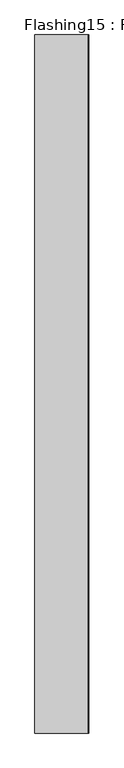
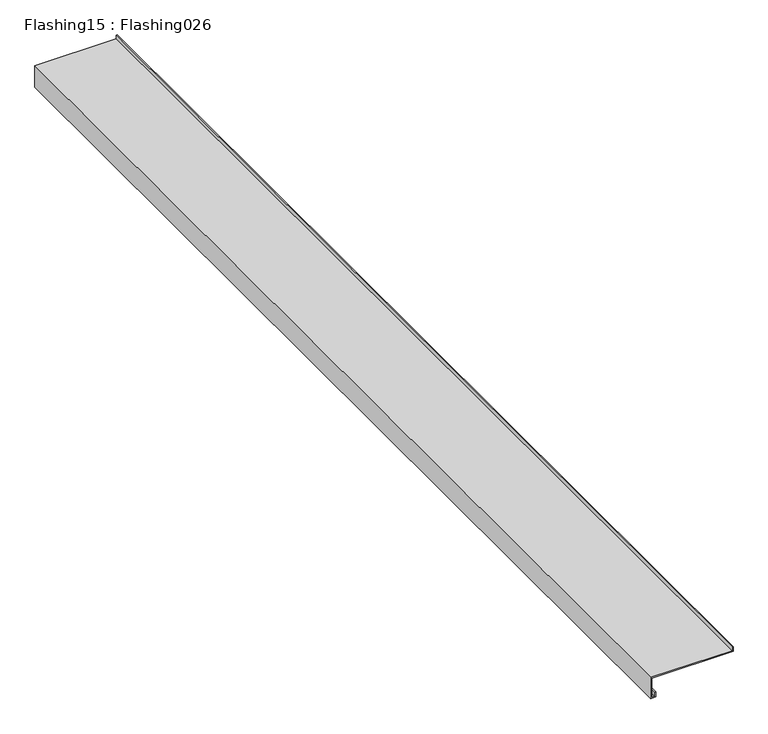
"""IFC4 building model written with IfcOpenShell, lengths in millimetres: proxy geometry, Flashing15 : Flashing026."""

from ifc_helpers import new_model, si_unit, frame, origin, place, context, project, spatial, polyline, outline, extrude, source, transform, mapped, element, save


def flashing15_flashing026_3ad6fd26(model_context):
    return source(origin(), model_context, "Body", "SweptSolid", [
        extrude(outline(polyline([(36566.1804687, -1997.9650879), (36558.9851563, -1997.9650879), (36558.9851563, -2150.7495117), (36516.8054688, -2150.7495117), (36516.8054688, -2140.6896973), (36527.3601562, -2140.6896973), (36527.3601562, -2142.6896973), (36518.8054687, -2142.6896973), (36518.8054687, -2148.7495117), (36556.9851562, -2148.7495117), (36556.9851562, -1995.9650879), (36566.1804687, -1995.9650879), (36566.1804687, -1997.9650879)])), frame((0.0, 998.1570053, 0.0), z_axis=(0.0, 1.0, 0.0), x_axis=(0.0, 0.0, 1.0)), (0.0, 0.0, 1.0), 2000.0),
    ])


if __name__ == "__main__":
    model = new_model("IFC4")
    model_context = context("Model", 3, world=origin())
    ifc_project = project(units=[si_unit("LENGTHUNIT", "METRE", prefix="MILLI")], contexts=[model_context])
    site = spatial("IfcSite", under=ifc_project)
    building = spatial("IfcBuilding", under=site)
    placement = place(None, origin())
    flashing15_flashing026_shape = flashing15_flashing026_3ad6fd26(model_context)
    element("IfcBuildingElementProxy", 1, Name="Flashing15 : Flashing026", ObjectType="Flashing15 : Flashing026", at=placement, inside=building, context=model_context, shape_type="MappedRepresentation", body=[
        mapped(flashing15_flashing026_shape, transform((0.0, 0.0, 0.0), x_axis=(1.0, 0.0, 0.0), y_axis=(0.0, 1.0, 0.0), z_axis=(0.0, 0.0, 1.0))),
    ])
    save(model, "model.ifc")

# Revit data of these elements
# Type "Flashing15 : Flashing026"
#   NameOverride = "Flashing026"
# Element 1 (IfcBuildingElementProxy, "Flashing15 : Flashing026")
#   Materials on its faces: "16GA. COPPER BRAKE METAL FLASHING"
# Materials
#   "16GA. COPPER BRAKE METAL FLASHING": class "Unassigned", colour RGB 128 128 128, transparency 0, Cost = 0
